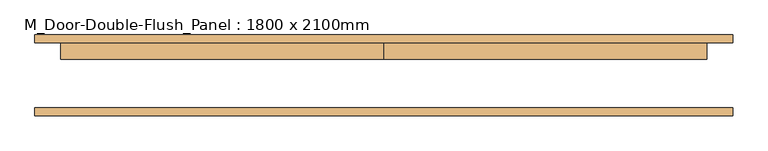
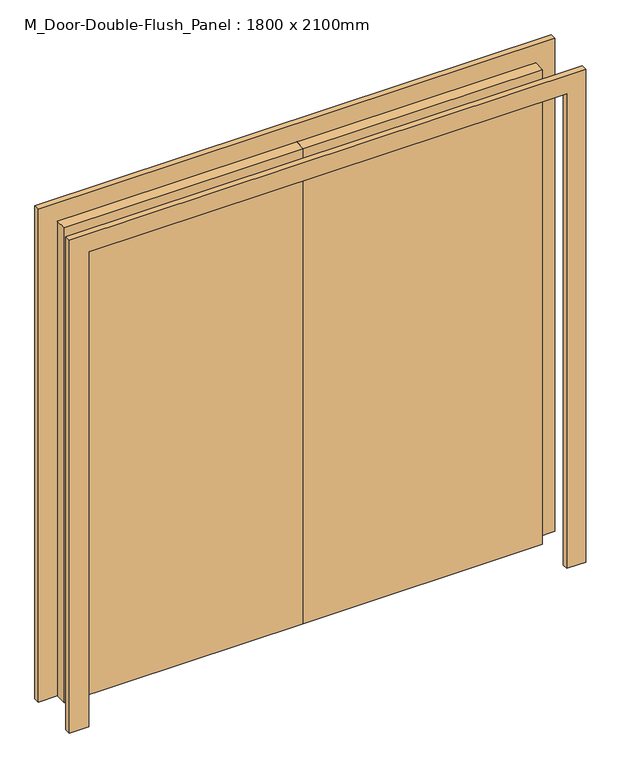
"""IFC4 building model written with IfcOpenShell, lengths in millimetres: door geometry, M_Door-Double-Flush_Panel : 1800 x 2100mm."""

import ifcopenshell
import ifcopenshell.guid

model = None  # the IFC model being written
_history = None  # IfcOwnerHistory: only IFC2X3 demands one
_inside = {}  # id of a spatial element -> (the spatial element, [elements in it])
_under = {}  # id of a project, library or spatial element -> (it, [spatial elements below it])
_declared = {}  # id of a project -> (the project, [libraries it declares])
_typed = {}  # id of a type object -> (the type object, [elements of that type])
_made_of = {}  # id of a material, layer set ... -> (it, [elements and type objects made of it])


def new_model(schema):
    """Start an empty IFC model of exactly this schema.

    Asked for "IFC4X3", IfcOpenShell would pick the latest addendum, in which some entities
    have other attributes; the version numbers below select the first issue.
    IFC2X3 requires an IfcOwnerHistory on every rooted entity: one is made here for all.
    """
    global model, _history
    if schema == "IFC4X3":
        model = ifcopenshell.file(schema_version=(4, 3, 0, 0))
    else:
        model = ifcopenshell.file(schema=schema)
    _inside.clear()
    _under.clear()
    _declared.clear()
    _typed.clear()
    _made_of.clear()
    _history = None
    if model.schema == "IFC2X3":
        org = make("IfcOrganization", Name="unknown")
        user = make(
            "IfcPersonAndOrganization",
            ThePerson=make("IfcPerson", FamilyName="unknown"),
            TheOrganization=org,
        )
        app = make(
            "IfcApplication",
            ApplicationDeveloper=org,
            Version="unknown",
            ApplicationFullName="unknown",
            ApplicationIdentifier="unknown",
        )
        _history = make(
            "IfcOwnerHistory",
            OwningUser=user,
            OwningApplication=app,
            ChangeAction="ADDED",
            CreationDate=0,
        )
    return model


def make(cls, **values):
    """One entity of the class cls with the attributes given. An attribute that is None is left unset."""
    return model.create_entity(
        cls, **{name: value for name, value in values.items() if value is not None}
    )


def rooted(cls, **values):
    """An entity with a GlobalId (a new one), such as an element, a storey or a relation."""
    return make(cls, GlobalId=ifcopenshell.guid.new(), OwnerHistory=_history, **values)


def si_unit(unit_type, name, prefix=None):
    """IfcSIUnit, for example si_unit("LENGTHUNIT", "METRE", prefix="MILLI")."""
    return make("IfcSIUnit", UnitType=unit_type, Prefix=prefix, Name=name)


def assignment(units):
    """IfcUnitAssignment: the units of a project."""
    return None if units is None else make("IfcUnitAssignment", Units=units)


def point(xyz):
    """IfcCartesianPoint."""
    return None if xyz is None else make("IfcCartesianPoint", Coordinates=xyz)


def direction(xyz):
    """IfcDirection."""
    return None if xyz is None else make("IfcDirection", DirectionRatios=xyz)


def frame(location, z_axis=None, x_axis=None):
    """IfcAxis2Placement3D, a coordinate frame: its origin and axes. An axis left out is left unset."""
    return make(
        "IfcAxis2Placement3D",
        Location=point(location),
        Axis=direction(z_axis),
        RefDirection=direction(x_axis),
    )


def origin():
    """The frame at (0, 0, 0) with its axes left unset."""
    return frame((0.0, 0.0, 0.0))


def origin_with_axes():
    """The frame at (0, 0, 0) with the z axis (0, 0, 1) and the x axis (1, 0, 0) written out."""
    return frame((0.0, 0.0, 0.0), z_axis=(0.0, 0.0, 1.0), x_axis=(1.0, 0.0, 0.0))


def place(relative_to, where):
    """IfcLocalPlacement: puts the frame where relative to a parent placement (None: the world)."""
    return make(
        "IfcLocalPlacement", PlacementRelTo=relative_to, RelativePlacement=where
    )


def context(
    kind, dimensions, precision=None, world=None, true_north=None, identifier=None
):
    """IfcGeometricRepresentationContext, for example the 3D "Model" context."""
    return make(
        "IfcGeometricRepresentationContext",
        ContextIdentifier=identifier,
        ContextType=kind,
        CoordinateSpaceDimension=dimensions,
        Precision=precision,
        WorldCoordinateSystem=world,
        TrueNorth=true_north,
    )


def project(units=None, contexts=None):
    """IfcProject with its units and contexts."""
    return rooted(
        "IfcProject",
        Name="project",
        RepresentationContexts=contexts,
        UnitsInContext=assignment(units),
    )


def spatial(cls, under=None, at=None, **own):
    """A site, building, storey or space (cls), placed at a placement, below another one or the project."""
    s = rooted(cls, ObjectPlacement=at, **own)
    if under is not None:
        _under.setdefault(under.id(), (under, []))[1].append(s)
    return s


def polyline(points):
    """IfcPolyline through the points."""
    return make("IfcPolyline", Points=[point(p) for p in points])


def outline(outer, holes=None, kind="AREA"):
    """IfcArbitraryClosedProfileDef: a profile drawn as a closed curve; with holes, ...WithVoids."""
    if holes is None:
        return make("IfcArbitraryClosedProfileDef", ProfileType=kind, OuterCurve=outer)
    return make(
        "IfcArbitraryProfileDefWithVoids",
        ProfileType=kind,
        OuterCurve=outer,
        InnerCurves=holes,
    )


def extrude(swept, where, along, depth):
    """IfcExtrudedAreaSolid: the profile swept, set in the frame where, extruded along a direction by depth."""
    return make(
        "IfcExtrudedAreaSolid",
        SweptArea=swept,
        Position=where,
        ExtrudedDirection=direction(along),
        Depth=depth,
    )


def shape(context_of_items, identifier, shape_type, items):
    """IfcShapeRepresentation: the items that make up one representation, for example the "Body"."""
    return make(
        "IfcShapeRepresentation",
        ContextOfItems=context_of_items,
        RepresentationIdentifier=identifier,
        RepresentationType=shape_type,
        Items=items,
    )


def source(mapping_origin, context_of_items, identifier, shape_type, items):
    """IfcRepresentationMap: a shape defined once, which mapped items show again and again."""
    return make(
        "IfcRepresentationMap",
        MappingOrigin=mapping_origin,
        MappedRepresentation=shape(context_of_items, identifier, shape_type, items),
    )


def transform(
    local_origin,
    x_axis=None,
    y_axis=None,
    z_axis=None,
    scale=None,
    scale2=None,
    scale3=None,
    uniform=True,
):
    """IfcCartesianTransformationOperator3D, or its non-uniform kind. x_axis, y_axis, z_axis: its Axis1, 2, 3."""
    if uniform:
        return make(
            "IfcCartesianTransformationOperator3D",
            Axis1=direction(x_axis),
            Axis2=direction(y_axis),
            LocalOrigin=point(local_origin),
            Scale=scale,
            Axis3=direction(z_axis),
        )
    return make(
        "IfcCartesianTransformationOperator3DnonUniform",
        Axis1=direction(x_axis),
        Axis2=direction(y_axis),
        LocalOrigin=point(local_origin),
        Scale=scale,
        Axis3=direction(z_axis),
        Scale2=scale2,
        Scale3=scale3,
    )


def mapped(mapping_source, mapping_target):
    """IfcMappedItem: shows the shape of a source again, moved by a transform."""
    return make(
        "IfcMappedItem", MappingSource=mapping_source, MappingTarget=mapping_target
    )


def made_of(thing, what):
    """Note that an element or type object is made of a material, layer set ...; save() writes the relation."""
    if what is not None:
        _made_of.setdefault(what.id(), (what, []))[1].append(thing)
    return thing


def element(
    cls,
    number,
    at=None,
    inside=None,
    cuts=None,
    type_object=None,
    material=None,
    context=None,
    identifier="Body",
    shape_type=None,
    held_by="IfcProductDefinitionShape",
    body=None,
    shapes=None,
    **own,
):
    """One element of the class cls, such as IfcWall. Its Tag is "e" and its number.

    at: its placement. inside: the storey or other place that contains it. cuts: it is an
    opening in that element (IfcRelVoidsElement). A single representation is given by context,
    identifier, shape_type and body (its items); several are given by shapes. held_by: the class
    of the entity that holds the representations. save() writes the other relations.
    """
    e = rooted(cls, Tag="e%d" % number, ObjectPlacement=at, **own)
    if body is not None:
        shapes = [shape(context, identifier, shape_type, body)]
    if shapes is not None:
        e.Representation = make(held_by, Representations=shapes)
    if inside is not None:
        _inside.setdefault(inside.id(), (inside, []))[1].append(e)
    if cuts is not None:
        rooted(
            "IfcRelVoidsElement", RelatingBuildingElement=cuts, RelatedOpeningElement=e
        )
    if type_object is not None:
        _typed.setdefault(type_object.id(), (type_object, []))[1].append(e)
    return made_of(e, material)


def aggregate(whole, parts):
    """IfcRelAggregates: a whole, such as a stair, and the parts it consists of."""
    return rooted("IfcRelAggregates", RelatingObject=whole, RelatedObjects=parts)


def save(model, path):
    """Write the relations noted so far, then the file.

    IfcRelAggregates (storeys below a building ...), IfcRelContainedInSpatialStructure (elements
    in a storey), IfcRelDefinesByType, IfcRelAssociatesMaterial and IfcRelDeclares: one each for
    every whole, place, type object, material and project.
    """
    for whole, parts in _under.values():
        aggregate(whole, parts)
    for where, things in _inside.values():
        rooted(
            "IfcRelContainedInSpatialStructure",
            RelatedElements=things,
            RelatingStructure=where,
        )
    for kind, things in _typed.values():
        rooted("IfcRelDefinesByType", RelatedObjects=things, RelatingType=kind)
    for what, things in _made_of.values():
        rooted("IfcRelAssociatesMaterial", RelatedObjects=things, RelatingMaterial=what)
    for by, libraries in _declared.values():
        rooted("IfcRelDeclares", RelatingContext=by, RelatedDefinitions=libraries)
    model.write(path)


def m_door_double_flush_panel_1800_x_2100mm_345fcf8f(model_context):
    return source(origin(), model_context, "Body", "SweptSolid", [
        extrude(outline(polyline([(2100.0, -1000.0), (2100.0, 1000.0), (0.0, 1000.0), (0.0, 1080.0), (2180.0, 1080.0), (2180.0, -1080.0), (0.0, -1080.0), (0.0, -1000.0), (2100.0, -1000.0)])), frame((0.0, -125.0, 0.0), z_axis=(0.0, 1.0, 0.0), x_axis=(0.0, 0.0, 1.0)), (0.0, 0.0, 1.0), 25.0),
        extrude(outline(polyline([(2100.0, -1000.0), (2100.0, 1000.0), (0.0, 1000.0), (0.0, 1080.0), (2180.0, 1080.0), (2180.0, -1080.0), (0.0, -1080.0), (0.0, -1000.0), (2100.0, -1000.0)])), frame((0.0, 100.0, 0.0), z_axis=(0.0, 1.0, 0.0), x_axis=(0.0, 0.0, 1.0)), (0.0, 0.0, 1.0), 25.0),
        extrude(outline(polyline([(0.0, 100.0), (1000.0, 100.0), (1000.0, 50.0), (0.0, 50.0), (0.0, 100.0)])), origin_with_axes(), (0.0, 0.0, 1.0), 2100.0),
        extrude(outline(polyline([(-1000.0, 100.0), (0.0, 100.0), (0.0, 50.0), (-1000.0, 50.0), (-1000.0, 100.0)])), origin_with_axes(), (0.0, 0.0, 1.0), 2100.0),
    ])


if __name__ == "__main__":
    model = new_model("IFC4")
    model_context = context("Model", 3, world=origin())
    ifc_project = project(units=[si_unit("LENGTHUNIT", "METRE", prefix="MILLI")], contexts=[model_context])
    site = spatial("IfcSite", under=ifc_project)
    building = spatial("IfcBuilding", under=site)
    placement = place(None, origin())
    m_door_double_flush_panel_1800_x_2100mm_shape = m_door_double_flush_panel_1800_x_2100mm_345fcf8f(model_context)
    element("IfcDoor", 1, ObjectType="M_Door-Double-Flush_Panel : 1800 x 2100mm", at=placement, inside=building, context=model_context, shape_type="MappedRepresentation", body=[
        mapped(m_door_double_flush_panel_1800_x_2100mm_shape, transform((0.0, 0.0, 0.0), x_axis=(1.0, 0.0, 0.0), y_axis=(0.0, 1.0, 0.0), z_axis=(0.0, 0.0, 1.0))),
    ])
    save(model, "model.ifc")

# Revit data of these elements
# Type "M_Door-Double-Flush_Panel : 1800 x 2100mm"
#   Type Mark = "22"
#   Construction Type Id = "DOOR"
#   Assembly Code = "C1020"
#   Analytic Construction = "Wooden"
#   Thickness = 0.05 m
#   Thermal Resistance (R) = 0.455703 (m²·K)/W
#   Swing Angle [instance default] = 90.00°
#   Panel Width = 1 m
#   Heat Transfer Coefficient (U) = 2.19465 W/(m²·K)
#   Height = 2.1 m
#   Trim Projection Ext = 0.025 m
#   Trim Projection Int = 0.025 m
#   Trim Width = 0.08 m
#   Width = 2 m
#   Panel Material = Glass
#   Trim Material = bordes
#   Visual Light Transmittance = 0
#   Solar Heat Gain Coefficient = 0
#   Function = (empty or 0)
#   Wall Closure = (empty or 0)
# Element 1 (IfcDoor, "M_Door-Double-Flush_Panel : 1800 x 2100mm")
#   Materials on its faces: "bordes", "Glass"
# Materials
#   "Glass": class "Glass", colour RGB 218 227 224, transparency 0.85, Description = "Soda Lime Glass", Cost = 0
#   "bordes": class "Generic", colour RGB 56 56 56, transparency 0, Cost = 0
